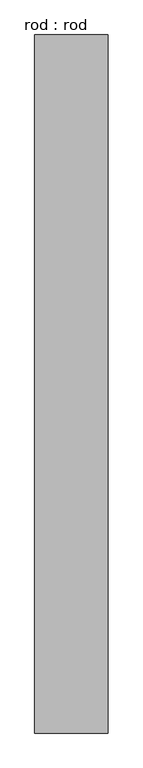
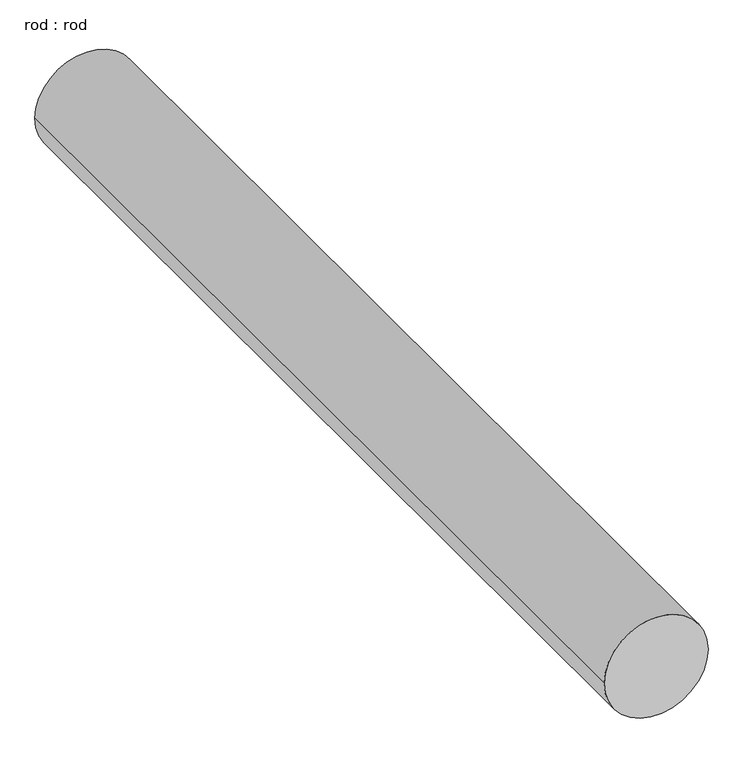
"""IFC4 building model written with IfcOpenShell, lengths in millimetres: proxy geometry, rod : rod."""

from ifc_helpers import new_model, si_unit, point, frame, frame_2d, origin, place, context, project, spatial, circle_curve, trimmed, segment, composite_curve, outline, extrude, source, transform, mapped, element, save


def rod_rod_77116452(model_context):
    return source(origin(), model_context, "Body", "SweptSolid", [
        extrude(outline(composite_curve([segment(trimmed(circle_curve(frame_2d((0.0108462, 0.0)), 200.0), [point((0.0108462, 200.0))], [point((0.0108462, -200.0))], False, "CARTESIAN"), True, "CONTINUOUS"), segment(trimmed(circle_curve(frame_2d((0.0108462, 0.0)), 200.0), [point((0.0108462, -200.0))], [point((0.0108462, 200.0))], False, "CARTESIAN"), True, "CONTINUOUS")], self_intersect=False)), frame((0.0, 2195.0042359, 0.0), z_axis=(0.0, 1.0, 0.0), x_axis=(0.0, 0.0, 1.0)), (0.0, 0.0, 1.0), 3795.448759),
    ])


if __name__ == "__main__":
    model = new_model("IFC4")
    model_context = context("Model", 3, world=origin())
    ifc_project = project(units=[si_unit("LENGTHUNIT", "METRE", prefix="MILLI")], contexts=[model_context])
    site = spatial("IfcSite", under=ifc_project)
    building = spatial("IfcBuilding", under=site)
    placement = place(None, origin())
    rod_rod_shape = rod_rod_77116452(model_context)
    element("IfcBuildingElementProxy", 1, Name="rod : rod", ObjectType="rod : rod", at=placement, inside=building, context=model_context, shape_type="MappedRepresentation", body=[
        mapped(rod_rod_shape, transform((0.0, 0.0, 0.0), x_axis=(1.0, 0.0, 0.0), y_axis=(0.0, 1.0, 0.0), z_axis=(0.0, 0.0, 1.0))),
    ])
    save(model, "model.ifc")

# Revit data of these elements
# Type "rod : rod"
#   Default Elevation = 0
